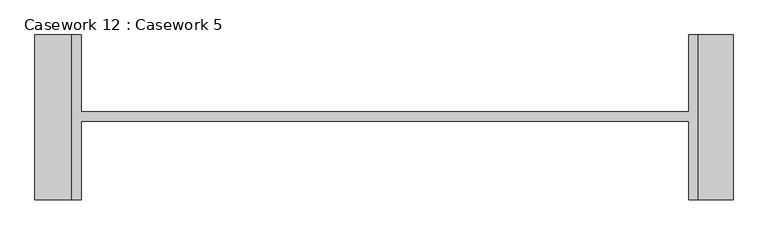
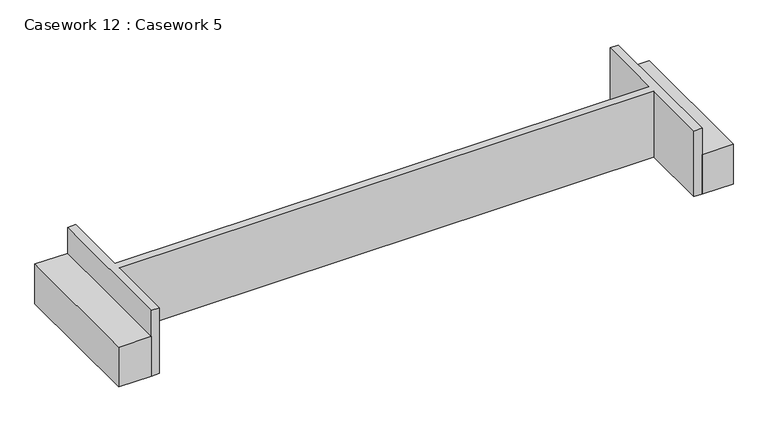
"""IFC4 building model written with IfcOpenShell, lengths in millimetres: furniture geometry, Casework 12 : Casework 5."""

import ifcopenshell
import ifcopenshell.guid

model = None  # the IFC model being written
_history = None  # IfcOwnerHistory: only IFC2X3 demands one
_inside = {}  # id of a spatial element -> (the spatial element, [elements in it])
_under = {}  # id of a project, library or spatial element -> (it, [spatial elements below it])
_declared = {}  # id of a project -> (the project, [libraries it declares])
_typed = {}  # id of a type object -> (the type object, [elements of that type])
_made_of = {}  # id of a material, layer set ... -> (it, [elements and type objects made of it])


def new_model(schema):
    """Start an empty IFC model of exactly this schema.

    Asked for "IFC4X3", IfcOpenShell would pick the latest addendum, in which some entities
    have other attributes; the version numbers below select the first issue.
    IFC2X3 requires an IfcOwnerHistory on every rooted entity: one is made here for all.
    """
    global model, _history
    if schema == "IFC4X3":
        model = ifcopenshell.file(schema_version=(4, 3, 0, 0))
    else:
        model = ifcopenshell.file(schema=schema)
    _inside.clear()
    _under.clear()
    _declared.clear()
    _typed.clear()
    _made_of.clear()
    _history = None
    if model.schema == "IFC2X3":
        org = make("IfcOrganization", Name="unknown")
        user = make(
            "IfcPersonAndOrganization",
            ThePerson=make("IfcPerson", FamilyName="unknown"),
            TheOrganization=org,
        )
        app = make(
            "IfcApplication",
            ApplicationDeveloper=org,
            Version="unknown",
            ApplicationFullName="unknown",
            ApplicationIdentifier="unknown",
        )
        _history = make(
            "IfcOwnerHistory",
            OwningUser=user,
            OwningApplication=app,
            ChangeAction="ADDED",
            CreationDate=0,
        )
    return model


def make(cls, **values):
    """One entity of the class cls with the attributes given. An attribute that is None is left unset."""
    return model.create_entity(
        cls, **{name: value for name, value in values.items() if value is not None}
    )


def rooted(cls, **values):
    """An entity with a GlobalId (a new one), such as an element, a storey or a relation."""
    return make(cls, GlobalId=ifcopenshell.guid.new(), OwnerHistory=_history, **values)


def si_unit(unit_type, name, prefix=None):
    """IfcSIUnit, for example si_unit("LENGTHUNIT", "METRE", prefix="MILLI")."""
    return make("IfcSIUnit", UnitType=unit_type, Prefix=prefix, Name=name)


def assignment(units):
    """IfcUnitAssignment: the units of a project."""
    return None if units is None else make("IfcUnitAssignment", Units=units)


def point(xyz):
    """IfcCartesianPoint."""
    return None if xyz is None else make("IfcCartesianPoint", Coordinates=xyz)


def direction(xyz):
    """IfcDirection."""
    return None if xyz is None else make("IfcDirection", DirectionRatios=xyz)


def frame(location, z_axis=None, x_axis=None):
    """IfcAxis2Placement3D, a coordinate frame: its origin and axes. An axis left out is left unset."""
    return make(
        "IfcAxis2Placement3D",
        Location=point(location),
        Axis=direction(z_axis),
        RefDirection=direction(x_axis),
    )


def origin():
    """The frame at (0, 0, 0) with its axes left unset."""
    return frame((0.0, 0.0, 0.0))


def origin_with_axes():
    """The frame at (0, 0, 0) with the z axis (0, 0, 1) and the x axis (1, 0, 0) written out."""
    return frame((0.0, 0.0, 0.0), z_axis=(0.0, 0.0, 1.0), x_axis=(1.0, 0.0, 0.0))


def place(relative_to, where):
    """IfcLocalPlacement: puts the frame where relative to a parent placement (None: the world)."""
    return make(
        "IfcLocalPlacement", PlacementRelTo=relative_to, RelativePlacement=where
    )


def context(
    kind, dimensions, precision=None, world=None, true_north=None, identifier=None
):
    """IfcGeometricRepresentationContext, for example the 3D "Model" context."""
    return make(
        "IfcGeometricRepresentationContext",
        ContextIdentifier=identifier,
        ContextType=kind,
        CoordinateSpaceDimension=dimensions,
        Precision=precision,
        WorldCoordinateSystem=world,
        TrueNorth=true_north,
    )


def project(units=None, contexts=None):
    """IfcProject with its units and contexts."""
    return rooted(
        "IfcProject",
        Name="project",
        RepresentationContexts=contexts,
        UnitsInContext=assignment(units),
    )


def spatial(cls, under=None, at=None, **own):
    """A site, building, storey or space (cls), placed at a placement, below another one or the project."""
    s = rooted(cls, ObjectPlacement=at, **own)
    if under is not None:
        _under.setdefault(under.id(), (under, []))[1].append(s)
    return s


def polyline(points):
    """IfcPolyline through the points."""
    return make("IfcPolyline", Points=[point(p) for p in points])


def outline(outer, holes=None, kind="AREA"):
    """IfcArbitraryClosedProfileDef: a profile drawn as a closed curve; with holes, ...WithVoids."""
    if holes is None:
        return make("IfcArbitraryClosedProfileDef", ProfileType=kind, OuterCurve=outer)
    return make(
        "IfcArbitraryProfileDefWithVoids",
        ProfileType=kind,
        OuterCurve=outer,
        InnerCurves=holes,
    )


def extrude(swept, where, along, depth):
    """IfcExtrudedAreaSolid: the profile swept, set in the frame where, extruded along a direction by depth."""
    return make(
        "IfcExtrudedAreaSolid",
        SweptArea=swept,
        Position=where,
        ExtrudedDirection=direction(along),
        Depth=depth,
    )


def shape(context_of_items, identifier, shape_type, items):
    """IfcShapeRepresentation: the items that make up one representation, for example the "Body"."""
    return make(
        "IfcShapeRepresentation",
        ContextOfItems=context_of_items,
        RepresentationIdentifier=identifier,
        RepresentationType=shape_type,
        Items=items,
    )


def source(mapping_origin, context_of_items, identifier, shape_type, items):
    """IfcRepresentationMap: a shape defined once, which mapped items show again and again."""
    return make(
        "IfcRepresentationMap",
        MappingOrigin=mapping_origin,
        MappedRepresentation=shape(context_of_items, identifier, shape_type, items),
    )


def transform(
    local_origin,
    x_axis=None,
    y_axis=None,
    z_axis=None,
    scale=None,
    scale2=None,
    scale3=None,
    uniform=True,
):
    """IfcCartesianTransformationOperator3D, or its non-uniform kind. x_axis, y_axis, z_axis: its Axis1, 2, 3."""
    if uniform:
        return make(
            "IfcCartesianTransformationOperator3D",
            Axis1=direction(x_axis),
            Axis2=direction(y_axis),
            LocalOrigin=point(local_origin),
            Scale=scale,
            Axis3=direction(z_axis),
        )
    return make(
        "IfcCartesianTransformationOperator3DnonUniform",
        Axis1=direction(x_axis),
        Axis2=direction(y_axis),
        LocalOrigin=point(local_origin),
        Scale=scale,
        Axis3=direction(z_axis),
        Scale2=scale2,
        Scale3=scale3,
    )


def mapped(mapping_source, mapping_target):
    """IfcMappedItem: shows the shape of a source again, moved by a transform."""
    return make(
        "IfcMappedItem", MappingSource=mapping_source, MappingTarget=mapping_target
    )


def made_of(thing, what):
    """Note that an element or type object is made of a material, layer set ...; save() writes the relation."""
    if what is not None:
        _made_of.setdefault(what.id(), (what, []))[1].append(thing)
    return thing


def element(
    cls,
    number,
    at=None,
    inside=None,
    cuts=None,
    type_object=None,
    material=None,
    context=None,
    identifier="Body",
    shape_type=None,
    held_by="IfcProductDefinitionShape",
    body=None,
    shapes=None,
    **own,
):
    """One element of the class cls, such as IfcWall. Its Tag is "e" and its number.

    at: its placement. inside: the storey or other place that contains it. cuts: it is an
    opening in that element (IfcRelVoidsElement). A single representation is given by context,
    identifier, shape_type and body (its items); several are given by shapes. held_by: the class
    of the entity that holds the representations. save() writes the other relations.
    """
    e = rooted(cls, Tag="e%d" % number, ObjectPlacement=at, **own)
    if body is not None:
        shapes = [shape(context, identifier, shape_type, body)]
    if shapes is not None:
        e.Representation = make(held_by, Representations=shapes)
    if inside is not None:
        _inside.setdefault(inside.id(), (inside, []))[1].append(e)
    if cuts is not None:
        rooted(
            "IfcRelVoidsElement", RelatingBuildingElement=cuts, RelatedOpeningElement=e
        )
    if type_object is not None:
        _typed.setdefault(type_object.id(), (type_object, []))[1].append(e)
    return made_of(e, material)


def aggregate(whole, parts):
    """IfcRelAggregates: a whole, such as a stair, and the parts it consists of."""
    return rooted("IfcRelAggregates", RelatingObject=whole, RelatedObjects=parts)


def save(model, path):
    """Write the relations noted so far, then the file.

    IfcRelAggregates (storeys below a building ...), IfcRelContainedInSpatialStructure (elements
    in a storey), IfcRelDefinesByType, IfcRelAssociatesMaterial and IfcRelDeclares: one each for
    every whole, place, type object, material and project.
    """
    for whole, parts in _under.values():
        aggregate(whole, parts)
    for where, things in _inside.values():
        rooted(
            "IfcRelContainedInSpatialStructure",
            RelatedElements=things,
            RelatingStructure=where,
        )
    for kind, things in _typed.values():
        rooted("IfcRelDefinesByType", RelatedObjects=things, RelatingType=kind)
    for what, things in _made_of.values():
        rooted("IfcRelAssociatesMaterial", RelatedObjects=things, RelatingMaterial=what)
    for by, libraries in _declared.values():
        rooted("IfcRelDeclares", RelatingContext=by, RelatedDefinitions=libraries)
    model.write(path)


def casework_12_casework_5_6038fc15(model_context):
    return source(origin(), model_context, "Body", "SweptSolid", [
        extrude(outline(polyline([(-45222.23615, 264550.8000155), (-45222.23615, 262009.748706), (-45765.6431786, 262009.748706), (-45765.6431786, 264550.8000155), (-45222.23615, 264550.8000155)])), origin_with_axes(), (0.0, 0.0, 1.0), 736.6),
        extrude(outline(polyline([(-55407.3218514, 264550.8000155), (-55407.3218514, 262009.748706), (-55978.0010565, 262009.748706), (-55978.0010565, 264550.8000155), (-55407.3218514, 264550.8000155)])), origin_with_axes(), (0.0, 0.0, 1.0), 736.6),
        extrude(outline(polyline([(-55264.4443999, 264550.8000155), (-55264.4443999, 263363.5915012), (-45907.3606126, 263363.5915012), (-45907.3606126, 264550.8000155), (-45765.6431786, 264550.8000155), (-45765.6431786, 262009.748706), (-45907.3606126, 262009.748706), (-45907.3606126, 263221.7281826), (-55264.4443999, 263221.7281826), (-55264.4443999, 262009.748706), (-55407.3218514, 262009.748706), (-55407.3218514, 264550.8000155), (-55264.4443999, 264550.8000155)])), origin_with_axes(), (0.0, 0.0, 1.0), 1219.2),
    ])


if __name__ == "__main__":
    model = new_model("IFC4")
    model_context = context("Model", 3, world=origin())
    ifc_project = project(units=[si_unit("LENGTHUNIT", "METRE", prefix="MILLI")], contexts=[model_context])
    site = spatial("IfcSite", under=ifc_project)
    building = spatial("IfcBuilding", under=site)
    placement = place(None, origin())
    casework_12_casework_5_shape = casework_12_casework_5_6038fc15(model_context)
    element("IfcFurniture", 1, ObjectType="Casework 12 : Casework 5", at=placement, inside=building, context=model_context, shape_type="MappedRepresentation", body=[
        mapped(casework_12_casework_5_shape, transform((0.0, 0.0, 0.0), x_axis=(1.0, 0.0, 0.0), y_axis=(0.0, 1.0, 0.0), z_axis=(0.0, 0.0, 1.0))),
    ])
    save(model, "model.ifc")

# Revit data of these elements
# Element 1 (IfcFurniture, "Casework 12 : Casework 5")
#   Materials on its faces: "Casework-oakfire"
# Materials
#   "Casework-oakfire": class "Miscellaneous", colour RGB 164 164 164, transparency 0, Cost = 0
